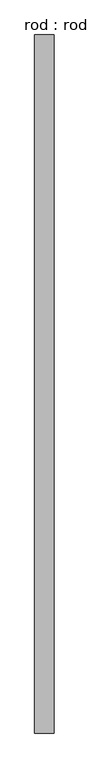
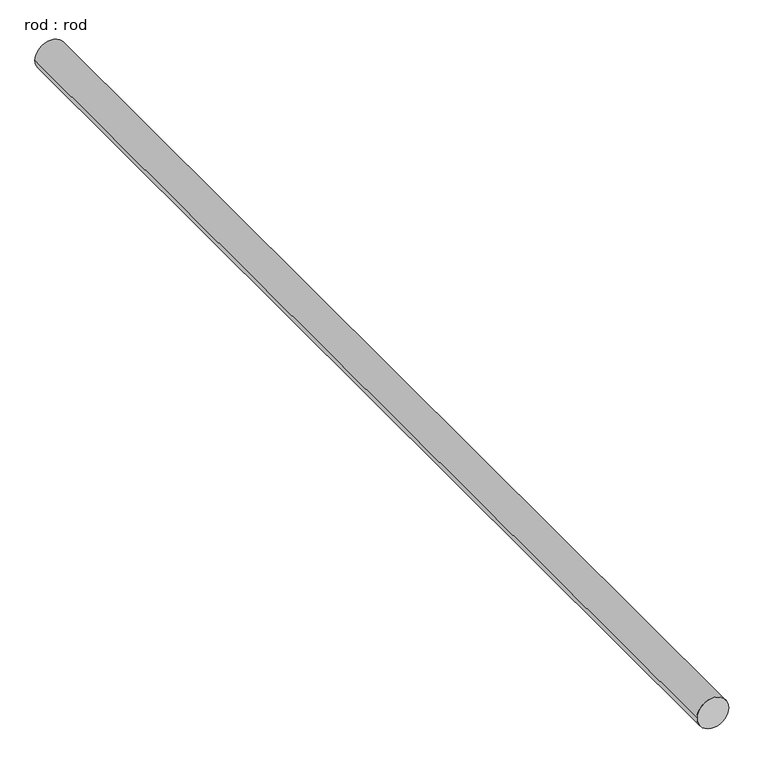
"""IFC4 building model written with IfcOpenShell, lengths in millimetres: proxy geometry, rod : rod."""

from ifc_helpers import new_model, si_unit, point, frame, frame_2d, origin, place, context, project, spatial, circle_curve, trimmed, segment, composite_curve, outline, extrude, source, transform, mapped, element, save


def rod_rod_92dcf860(model_context):
    return source(origin(), model_context, "Body", "SweptSolid", [
        extrude(outline(composite_curve([segment(trimmed(circle_curve(frame_2d((0.0108462, 0.0)), 200.0), [point((0.0108462, 200.0))], [point((0.0108462, -200.0))], False, "CARTESIAN"), True, "CONTINUOUS"), segment(trimmed(circle_curve(frame_2d((0.0108462, 0.0)), 200.0), [point((0.0108462, -200.0))], [point((0.0108462, 200.0))], False, "CARTESIAN"), True, "CONTINUOUS")], self_intersect=False)), frame((0.0, -3157.2713847, 0.0), z_axis=(0.0, 1.0, 0.0), x_axis=(0.0, 0.0, 1.0)), (0.0, 0.0, 1.0), 14500.0),
    ])


if __name__ == "__main__":
    model = new_model("IFC4")
    model_context = context("Model", 3, world=origin())
    ifc_project = project(units=[si_unit("LENGTHUNIT", "METRE", prefix="MILLI")], contexts=[model_context])
    site = spatial("IfcSite", under=ifc_project)
    building = spatial("IfcBuilding", under=site)
    placement = place(None, origin())
    rod_rod_shape = rod_rod_92dcf860(model_context)
    element("IfcBuildingElementProxy", 1, Name="rod : rod", ObjectType="rod : rod", at=placement, inside=building, context=model_context, shape_type="MappedRepresentation", body=[
        mapped(rod_rod_shape, transform((0.0, 0.0, 0.0), x_axis=(1.0, 0.0, 0.0), y_axis=(0.0, 1.0, 0.0), z_axis=(0.0, 0.0, 1.0))),
    ])
    save(model, "model.ifc")

# Revit data of these elements
# Type "rod : rod"
#   Default Elevation = 0
